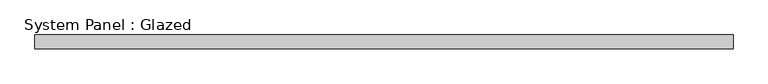
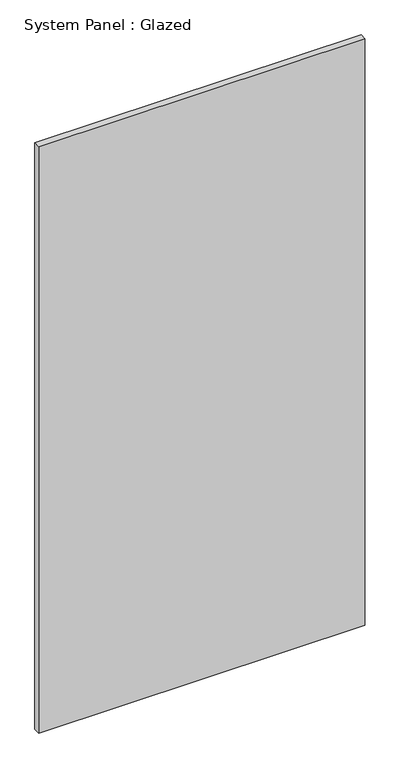
"""IFC4 building model written with IfcOpenShell, lengths in millimetres: plate geometry, System Panel : Glazed."""

from ifc_helpers import new_model, si_unit, origin, origin_with_axes, place, context, project, spatial, polyline, outline, extrude, source, transform, mapped, element, save


def system_panel_glazed_be4d4444(model_context):
    return source(origin(), model_context, "Body", "SweptSolid", [
        extrude(outline(polyline([(637.5, 24.5), (-637.5, 24.5), (-637.5, 49.5), (637.5, 49.5), (637.5, 24.5)])), origin_with_axes(), (0.0, 0.0, 1.0), 2422.0381538),
    ])


if __name__ == "__main__":
    model = new_model("IFC4")
    model_context = context("Model", 3, world=origin())
    ifc_project = project(units=[si_unit("LENGTHUNIT", "METRE", prefix="MILLI")], contexts=[model_context])
    site = spatial("IfcSite", under=ifc_project)
    building = spatial("IfcBuilding", under=site)
    placement = place(None, origin())
    system_panel_glazed_shape = system_panel_glazed_be4d4444(model_context)
    element("IfcPlate", 1, ObjectType="System Panel : Glazed", at=placement, inside=building, context=model_context, shape_type="MappedRepresentation", body=[
        mapped(system_panel_glazed_shape, transform((0.0, 0.0, 0.0), x_axis=(1.0, 0.0, 0.0), y_axis=(0.0, 1.0, 0.0), z_axis=(0.0, 0.0, 1.0))),
    ])
    save(model, "model.ifc")

# Revit data of these elements
# Type "System Panel : Glazed"
#   Keynote = "H11"
#   Construction Type Id = "GSP4R"
#   Analytic Construction = "1/8 in Pilkington single glazing"
#   Visual Light Transmittance = 0.9
#   Solar Heat Gain Coefficient = 0.86
#   Heat Transfer Coefficient (U) = 6.7069 W/(m²·K)
#   Define Thermal Properties by = 1
# Element 1 (IfcPlate, "System Panel : Glazed")
#   Materials on its faces: "Glass"
# Materials
#   "Glass": class "Glass", colour RGB 0 128 192, transparency 0.9, Description = "Soda Lime Glass", Cost = 0
